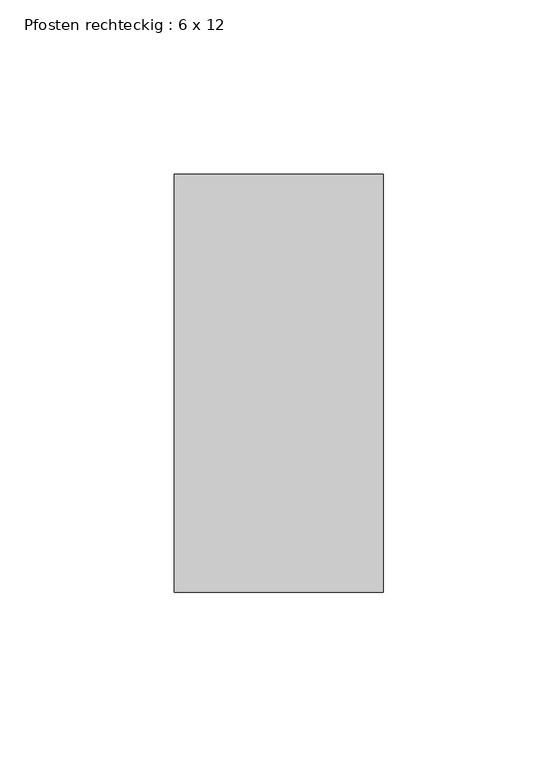
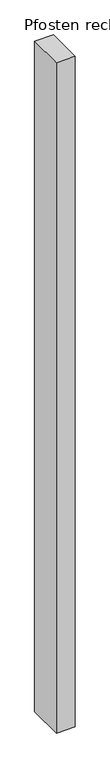
"""IFC4 building model written with IfcOpenShell, lengths in millimetres: member geometry, Pfosten rechteckig : 6 x 12."""

from ifc_helpers import new_model, si_unit, frame, origin, place, context, project, spatial, polyline, outline, extrude, source, transform, mapped, element, save


def pfosten_rechteckig_6_x_12_09906e8b(model_context):
    return source(origin(), model_context, "Body", "SweptSolid", [
        extrude(outline(polyline([(30.0, 60.0), (30.0, -60.0), (-30.0, -60.0), (-30.0, 60.0), (30.0, 60.0)])), frame((0.0, 0.0, -2264.8398838), z_axis=(0.0, 0.0, 1.0), x_axis=(1.0, 0.0, 0.0)), (0.0, 0.0, 1.0), 2264.8398838),
    ])


if __name__ == "__main__":
    model = new_model("IFC4")
    model_context = context("Model", 3, world=origin())
    ifc_project = project(units=[si_unit("LENGTHUNIT", "METRE", prefix="MILLI")], contexts=[model_context])
    site = spatial("IfcSite", under=ifc_project)
    building = spatial("IfcBuilding", under=site)
    placement = place(None, origin())
    pfosten_rechteckig_6_x_12_shape = pfosten_rechteckig_6_x_12_09906e8b(model_context)
    element("IfcMember", 1, ObjectType="Pfosten rechteckig : 6 x 12", at=placement, inside=building, context=model_context, shape_type="MappedRepresentation", body=[
        mapped(pfosten_rechteckig_6_x_12_shape, transform((0.0, 0.0, 0.0), x_axis=(1.0, 0.0, 0.0), y_axis=(0.0, 1.0, 0.0), z_axis=(0.0, 0.0, 1.0))),
    ])
    save(model, "model.ifc")

# Revit data of these elements
# Type "Pfosten rechteckig : 6 x 12"
#   built-in parameter 1007304 = 0.393701 (stored number, unit not read)
#   built-in parameter 1007301 = 0.0984252 (stored number, unit not read)
#   built-in parameter 1007300 = 0.0984252 (stored number, unit not read)
# Element 1 (IfcMember, "Pfosten rechteckig : 6 x 12")
#   Materials on its faces: "Metall - verzinkt"
# Materials
#   "Metall - verzinkt": class "Allgemeines", colour RGB 200 200 200, transparency 0, Cost = 0
